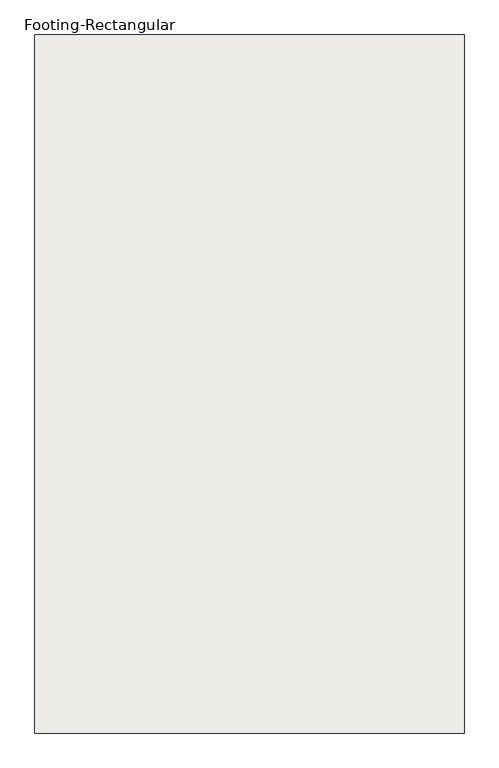
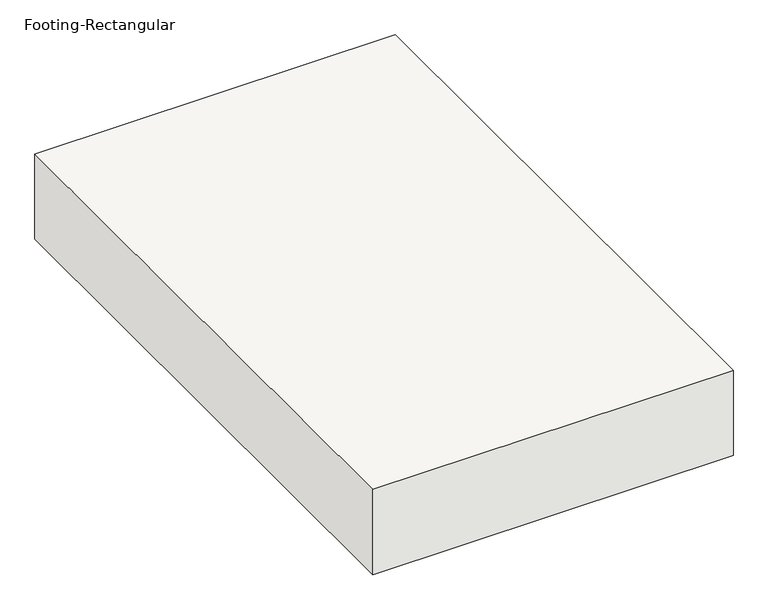
"""IFC4 building model written with IfcOpenShell, lengths in millimetres: slab geometry, Footing-Rectangular."""

from ifc_helpers import new_model, si_unit, frame, origin, place, context, project, spatial, polyline, outline, extrude, source, transform, mapped, element, save


def footing_rectangular_1b3ddeb7(model_context):
    return source(origin(), model_context, "Body", "SweptSolid", [
        extrude(outline(polyline([(1219.2, -1981.2), (-1219.2, -1981.2), (-1219.2, 1981.2), (1219.2, 1981.2), (1219.2, -1981.2)])), frame((0.0, 0.0, -609.6), z_axis=(0.0, 0.0, 1.0), x_axis=(1.0, 0.0, 0.0)), (0.0, 0.0, 1.0), 609.6),
    ])


if __name__ == "__main__":
    model = new_model("IFC4")
    model_context = context("Model", 3, world=origin())
    ifc_project = project(units=[si_unit("LENGTHUNIT", "METRE", prefix="MILLI")], contexts=[model_context])
    site = spatial("IfcSite", under=ifc_project)
    building = spatial("IfcBuilding", under=site)
    placement = place(None, origin())
    footing_rectangular_shape = footing_rectangular_1b3ddeb7(model_context)
    element("IfcSlab", 1, ObjectType="Footing-Rectangular : 8''-0\" x 13'-0\"", at=placement, inside=building, context=model_context, shape_type="MappedRepresentation", body=[
        mapped(footing_rectangular_shape, transform((0.0, 0.0, 0.0), x_axis=(1.0, 0.0, 0.0), y_axis=(0.0, 1.0, 0.0), z_axis=(0.0, 0.0, 1.0))),
    ])
    save(model, "model.ifc")

# Revit data of these elements
# Type "Footing-Rectangular : 8''-0\" x 13'-0\""
#   Assembly Code = "A1010100"
#   Width = 8' - 0"
#   Length = 13' - 0"
#   Thickness = 2' - 0"
#   Footing Material [instance default] = Concrete - Cast-in-Place Concrete
# Element 1 (IfcSlab, "Footing-Rectangular : 8''-0\" x 13'-0\"")
#   Materials on its faces: "Concrete - Cast-in-Place Concrete"
# Materials
#   "Concrete - Cast-in-Place Concrete": class "Concrete", colour RGB 192 192 192, transparency 0.4
